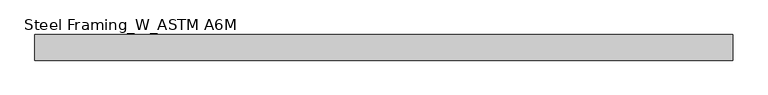
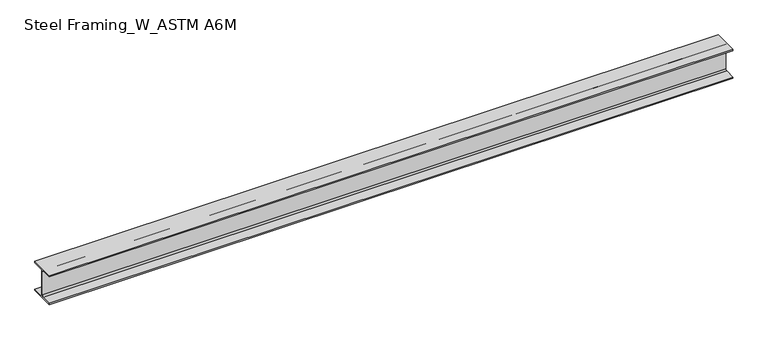
"""IFC4 building model written with IfcOpenShell, lengths in millimetres: beam geometry, Steel Framing_W_ASTM A6M : H_SB_AR_S02_W250x49.1_G5."""

from ifc_helpers import new_model, si_unit, point, frame, frame_2d, origin, place, context, project, spatial, polyline, circle_curve, trimmed, segment, composite_curve, outline, extrude, source, transform, mapped, element, save


def steel_framing_w_astm_a6m_e877a86a(model_context):
    return source(origin(), model_context, "Body", "SweptSolid", [
        extrude(outline(composite_curve([segment(polyline([(101.0, -112.5), (101.0, -123.5), (-101.0, -123.5), (-101.0, -112.5), (-16.385, -112.5)]), True, "CONTINUOUS"), segment(trimmed(circle_curve(frame_2d((-16.385, -99.8)), 12.7), [point((-16.385, -112.5))], [point((-3.685, -99.8))], True, "CARTESIAN"), True, "CONTINUOUS"), segment(polyline([(-3.685, -99.8), (-3.685, 99.8)]), True, "CONTINUOUS"), segment(trimmed(circle_curve(frame_2d((-16.385, 99.8)), 12.7), [point((-3.685, 99.8))], [point((-16.385, 112.5))], True, "CARTESIAN"), True, "CONTINUOUS"), segment(polyline([(-16.385, 112.5), (-101.0, 112.5), (-101.0, 123.5), (101.0, 123.5), (101.0, 112.5), (16.385, 112.5)]), True, "CONTINUOUS"), segment(trimmed(circle_curve(frame_2d((16.385, 99.8)), 12.7), [point((16.385, 112.5))], [point((3.685, 99.8))], True, "CARTESIAN"), True, "CONTINUOUS"), segment(polyline([(3.685, 99.8), (3.685, -99.8)]), True, "CONTINUOUS"), segment(trimmed(circle_curve(frame_2d((16.385, -99.8)), 12.7), [point((3.685, -99.8))], [point((16.385, -112.5))], True, "CARTESIAN"), True, "CONTINUOUS"), segment(polyline([(16.385, -112.5), (101.0, -112.5)]), True, "CONTINUOUS")], self_intersect=False)), frame((-2753.7, 0.0, 0.0), z_axis=(1.0, 0.0, 0.0), x_axis=(0.0, 1.0, 0.0)), (0.0, 0.0, 1.0), 5507.4),
    ])


if __name__ == "__main__":
    model = new_model("IFC4")
    model_context = context("Model", 3, world=origin())
    ifc_project = project(units=[si_unit("LENGTHUNIT", "METRE", prefix="MILLI")], contexts=[model_context])
    site = spatial("IfcSite", under=ifc_project)
    building = spatial("IfcBuilding", under=site)
    placement = place(None, origin())
    steel_framing_w_astm_a6m_shape = steel_framing_w_astm_a6m_e877a86a(model_context)
    element("IfcBeam", 1, ObjectType="Steel Framing_W_ASTM A6M : H_SB_AR_S02_W250x49.1_G5", at=placement, inside=building, context=model_context, shape_type="MappedRepresentation", body=[
        mapped(steel_framing_w_astm_a6m_shape, transform((0.0, 0.0, 0.0), x_axis=(1.0, 0.0, 0.0), y_axis=(0.0, 1.0, 0.0), z_axis=(0.0, 0.0, 1.0))),
    ])
    save(model, "model.ifc")

# Revit data of these elements
# Type "Steel Framing_W_ASTM A6M : H_SB_AR_S02_W250x49.1_G5"
#   Type Mark = "G5"
#   Section Name Key = "W10x33"
#   Width = 20.2 cm
#   Web Thickness = 0.737 cm
#   Web Fillet = 1.27 cm
#   Warping Constant = 212000.0 cm⁶
#   Torsional Moment of Inertia = 24.30 cm⁴
#   Section Area = 62.6 cm²
#   Plastic Modulus weak axis = 229.0 cm³
#   Plastic Modulus strong axis = 636.0 cm³
#   Perimeter = 1.27 m²/m
#   Nominal Weight = 49.10 kgf/m
#   Moment of Inertia weak axis = 1520.00 cm⁴
#   Moment of Inertia strong axis = 7120.00 cm⁴
#   Height = 24.7 cm
#   Flange Thickness = 1.1 cm
#   Elastic Modulus weak axis = 151.0 cm³
#   Elastic Modulus strong axis = 574.0 cm³
#   Centroid Vertical = 12.35 cm
#   Centroid Horizontal = 10.1 cm
#   Length [instance default] = 1500 mm
#   Structural Material [instance default] = Steel, 45-345
#   Bolt Spacing = 0
#   Assembly Code = ""
# Element 1 (IfcBeam, "Steel Framing_W_ASTM A6M : H_SB_AR_S02_W250x49.1_G5")
#   Materials on its faces: "Steel, 45-345"
# Materials
#   "Steel, 45-345": class "Metal", colour RGB 189 187 185, transparency 0, Description = "Steel 345 MPa", Cost = 0
